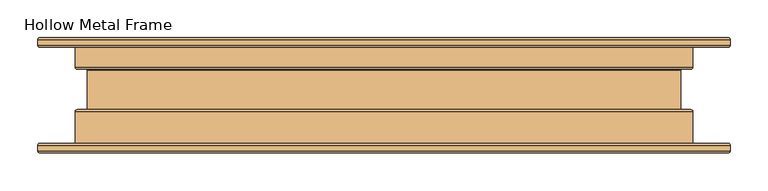
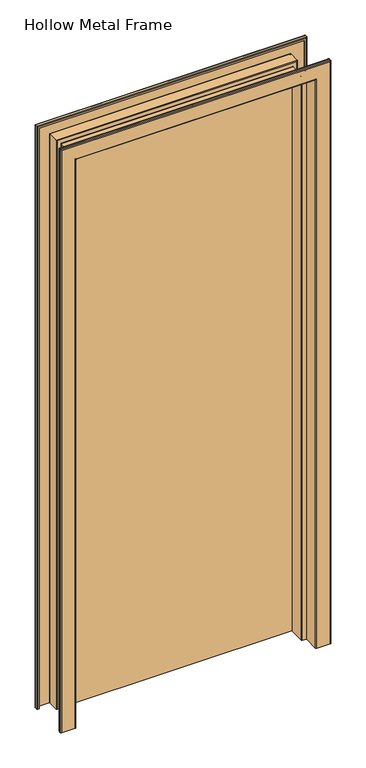
"""IFC4 building model written with IfcOpenShell, lengths in millimetres: door geometry, Hollow Metal Frame."""

from ifc_helpers import new_model, si_unit, frame, origin, origin_with_axes, place, context, project, spatial, polyline, circle_curve, ellipse_curve, outline, extrude, source, transform, mapped, element, save
from ifc_brep_helpers import plane_surface, cylinder_surface, revolved_surface, advanced_brep


def hollow_metal_frame_df2d566d(model_context):
    return source(origin(), model_context, "Body", "SolidModel", [
        advanced_brep(
        [(-454.62825, -63.5635, 0.0), (-449.2625, -63.5635, 0.0), (-449.2625, -65.11925, 0.0), (-454.62825, -65.11925, 0.0), (-455.64425, -66.13525, 0.0), (-455.64425, -73.66, 0.0), (-454.62825, -74.676, 0.0), (-408.97175, -74.676, 0.0), (-407.95575, -73.66, 0.0), (-407.95575, -21.68525, 0.0), (-405.384, -19.1135, 0.0), (-393.09675, -19.1135, 0.0), (-392.08075, -18.0975, 0.0), (-392.08075, 33.6931, 0.0), (-393.09675, 34.7091, 0.0), (-405.384, 34.7091, 0.0), (-407.95575, 37.28085, 0.0), (-407.95575, 73.5965, 0.0), (-408.97175, 74.6125, 0.0), (-454.62825, 74.6125, 0.0), (-455.64425, 73.5965, 0.0), (-455.64425, 66.07175, 0.0), (-454.62825, 65.05575, 0.0), (-449.2625, 65.05575, 0.0), (-449.2625, 63.5, 0.0), (-454.62825, 63.5, 0.0), (-457.2, 66.07175, 0.0), (-457.2, 73.5965, 0.0), (-454.62825, 76.16825, 0.0), (-408.97175, 76.16825, 0.0), (-406.4, 73.5965, 0.0), (-406.4, 37.28085, 0.0), (-405.384, 36.26485, 0.0), (-393.09675, 36.26485, 0.0), (-390.525, 33.6931, 0.0), (-390.525, -18.0975, 0.0), (-393.09675, -20.66925, 0.0), (-405.384, -20.66925, 0.0), (-406.4, -21.68525, 0.0), (-406.4, -73.66, 0.0), (-408.97175, -76.23175, 0.0), (-454.62825, -76.23175, 0.0), (-457.2, -73.66, 0.0), (-457.2, -66.13525, 0.0), (-457.2, -66.13525, 2082.8000001), (-454.62825, -63.5635, 2080.2282501), (-457.2, -73.66, 2082.8000001), (-454.62825, -76.23175, 2080.2282501), (-408.97175, -76.23175, 2034.5717501), (408.97175, -76.23175, 2034.5717501), (408.97175, -76.23175, 0.0), (454.62825, -76.23175, 0.0), (454.62825, -76.23175, 2080.2282501), (-406.4, -73.66, 2032.0000001), (-406.4, -21.68525, 2032.0000001), (-405.384, -20.66925, 2030.9840001), (-393.09675, -20.66925, 2018.6967501), (393.09675, -20.66925, 2018.6967501), (393.09675, -20.66925, 0.0), (405.384, -20.66925, 0.0), (405.384, -20.66925, 2030.9840001), (-390.525, -18.0975, 2016.1250001), (-390.525, 33.6931, 2016.1250001), (-393.09675, 36.26485, 2018.6967501), (-405.384, 36.26485, 2030.9840001), (405.384, 36.26485, 2030.9840001), (405.384, 36.26485, 0.0), (393.09675, 36.26485, 0.0), (393.09675, 36.26485, 2018.6967501), (-406.4, 37.28085, 2032.0000001), (-406.4, 73.5965, 2032.0000001), (-408.97175, 76.16825, 2034.5717501), (-454.62825, 76.16825, 2080.2282501), (454.62825, 76.16825, 2080.2282501), (454.62825, 76.16825, 0.0), (408.97175, 76.16825, 0.0), (408.97175, 76.16825, 2034.5717501), (-457.2, 73.5965, 2082.8000001), (-457.2, 66.07175, 2082.8000001), (-454.62825, 63.5, 2080.2282501), (-449.2625, 63.5, 2074.8625001), (449.2625, 63.5, 2074.8625001), (449.2625, 63.5, 0.0), (454.62825, 63.5, 0.0), (454.62825, 63.5, 2080.2282501), (-449.2625, 65.05575, 2074.8625001), (-454.62825, 65.05575, 2080.2282501), (454.62825, 65.05575, 2080.2282501), (454.62825, 65.05575, 0.0), (449.2625, 65.05575, 0.0), (449.2625, 65.05575, 2074.8625001), (-455.64425, 66.07175, 2081.2442501), (-455.64425, 73.5965, 2081.2442501), (-454.62825, 74.6125, 2080.2282501), (-408.97175, 74.6125, 2034.5717501), (408.97175, 74.6125, 2034.5717501), (408.97175, 74.6125, 0.0), (454.62825, 74.6125, 0.0), (454.62825, 74.6125, 2080.2282501), (-407.95575, 73.5965, 2033.5557501), (-407.95575, 37.28085, 2033.5557501), (-405.384, 34.7091, 2030.9840001), (-393.09675, 34.7091, 2018.6967501), (393.09675, 34.7091, 2018.6967501), (393.09675, 34.7091, 0.0), (405.384, 34.7091, 0.0), (405.384, 34.7091, 2030.9840001), (-392.08075, 33.6931, 2017.6807501), (-392.08075, -18.0975, 2017.6807501), (-393.09675, -19.1135, 2018.6967501), (-405.384, -19.1135, 2030.9840001), (405.384, -19.1135, 2030.9840001), (405.384, -19.1135, 0.0), (393.09675, -19.1135, 0.0), (393.09675, -19.1135, 2018.6967501), (-407.95575, -21.68525, 2033.5557501), (-407.95575, -73.66, 2033.5557501), (-408.97175, -74.676, 2034.5717501), (-454.62825, -74.676, 2080.2282501), (454.62825, -74.676, 2080.2282501), (454.62825, -74.676, 0.0), (408.97175, -74.676, 0.0), (408.97175, -74.676, 2034.5717501), (-455.64425, -73.66, 2081.2442501), (-455.64425, -66.13525, 2081.2442501), (-454.62825, -65.11925, 2080.2282501), (-449.2625, -65.11925, 2074.8625001), (449.2625, -65.11925, 2074.8625001), (449.2625, -65.11925, 0.0), (454.62825, -65.11925, 0.0), (454.62825, -65.11925, 2080.2282501), (-449.2625, -63.5635, 2074.8625001), (454.62825, -63.5635, 2080.2282501), (454.62825, -63.5635, 0.0), (449.2625, -63.5635, 0.0), (449.2625, -63.5635, 2074.8625001), (457.2, -66.13525, 2082.8000001), (457.2, -73.66, 2082.8000001), (406.4, -73.66, 2032.0000001), (406.4, -21.68525, 2032.0000001), (390.525, -18.0975, 2016.1250001), (390.525, 33.6931, 2016.1250001), (406.4, 37.28085, 2032.0000001), (406.4, 73.5965, 2032.0000001), (457.2, 73.5965, 2082.8000001), (457.2, 66.07175, 2082.8000001), (455.64425, 66.07175, 2081.2442501), (455.64425, 73.5965, 2081.2442501), (407.95575, 73.5965, 2033.5557501), (407.95575, 37.28085, 2033.5557501), (392.08075, 33.6931, 2017.6807501), (392.08075, -18.0975, 2017.6807501), (407.95575, -21.68525, 2033.5557501), (407.95575, -73.66, 2033.5557501), (455.64425, -73.66, 2081.2442501), (455.64425, -66.13525, 2081.2442501), (457.2, -66.13525, 0.0), (457.2, -73.66, 0.0), (406.4, -73.66, 0.0), (406.4, -21.68525, 0.0), (390.525, -18.0975, 0.0), (390.525, 33.6931, 0.0), (406.4, 37.28085, 0.0), (406.4, 73.5965, 0.0), (457.2, 73.5965, 0.0), (457.2, 66.07175, 0.0), (455.64425, 66.07175, 0.0), (455.64425, 73.5965, 0.0), (407.95575, 73.5965, 0.0), (407.95575, 37.28085, 0.0), (392.08075, 33.6931, 0.0), (392.08075, -18.0975, 0.0), (407.95575, -21.68525, 0.0), (407.95575, -73.66, 0.0), (455.64425, -73.66, 0.0), (455.64425, -66.13525, 0.0)],
        [
            (0, 1),
            (1, 2),
            (2, 3),
            (3, 4, circle_curve(frame((-454.62825, -66.13525, 0.0), z_axis=(0.0, 0.0, 1.0), x_axis=(0.0, 1.0, 0.0)), 1.016)),
            (4, 5),
            (5, 6, circle_curve(frame((-454.62825, -73.66, 0.0), z_axis=(0.0, 0.0, 1.0), x_axis=(0.0, 1.0, 0.0)), 1.016)),
            (6, 7),
            (7, 8, circle_curve(frame((-408.97175, -73.66, 0.0), z_axis=(0.0, 0.0, 1.0), x_axis=(0.0, 1.0, 0.0)), 1.016)),
            (8, 9),
            (9, 10, circle_curve(frame((-405.384, -21.68525, 0.0), z_axis=(0.0, 0.0, -1.0), x_axis=(0.0, 1.0, 0.0)), 2.57175)),
            (10, 11),
            (11, 12, circle_curve(frame((-393.09675, -18.0975, 0.0), z_axis=(0.0, 0.0, 1.0), x_axis=(0.0, 1.0, 0.0)), 1.016)),
            (12, 13),
            (13, 14, circle_curve(frame((-393.09675, 33.6931, 0.0), z_axis=(0.0, 0.0, 1.0), x_axis=(0.0, 1.0, 0.0)), 1.016)),
            (14, 15),
            (15, 16, circle_curve(frame((-405.384, 37.28085, 0.0), z_axis=(0.0, 0.0, -1.0), x_axis=(0.0, 1.0, 0.0)), 2.57175)),
            (16, 17),
            (17, 18, circle_curve(frame((-408.97175, 73.5965, 0.0), z_axis=(0.0, 0.0, 1.0), x_axis=(0.0, 1.0, 0.0)), 1.016)),
            (18, 19),
            (19, 20, circle_curve(frame((-454.62825, 73.5965, 0.0), z_axis=(0.0, 0.0, 1.0), x_axis=(0.0, 1.0, 0.0)), 1.016)),
            (20, 21),
            (21, 22, circle_curve(frame((-454.62825, 66.07175, 0.0), z_axis=(0.0, 0.0, 1.0), x_axis=(0.0, 1.0, 0.0)), 1.016)),
            (22, 23),
            (23, 24),
            (24, 25),
            (25, 26, circle_curve(frame((-454.62825, 66.07175, 0.0), z_axis=(0.0, 0.0, -1.0), x_axis=(0.0, 1.0, 0.0)), 2.57175)),
            (26, 27),
            (27, 28, circle_curve(frame((-454.62825, 73.5965, 0.0), z_axis=(0.0, 0.0, -1.0), x_axis=(0.0, 1.0, 0.0)), 2.57175)),
            (28, 29),
            (29, 30, circle_curve(frame((-408.97175, 73.5965, 0.0), z_axis=(0.0, 0.0, -1.0), x_axis=(0.0, 1.0, 0.0)), 2.57175)),
            (30, 31),
            (31, 32, circle_curve(frame((-405.384, 37.28085, 0.0), z_axis=(0.0, 0.0, 1.0), x_axis=(0.0, 1.0, 0.0)), 1.016)),
            (32, 33),
            (33, 34, circle_curve(frame((-393.09675, 33.6931, 0.0), z_axis=(0.0, 0.0, -1.0), x_axis=(0.0, 1.0, 0.0)), 2.57175)),
            (34, 35),
            (35, 36, circle_curve(frame((-393.09675, -18.0975, 0.0), z_axis=(0.0, 0.0, -1.0), x_axis=(0.0, 1.0, 0.0)), 2.57175)),
            (36, 37),
            (37, 38, circle_curve(frame((-405.384, -21.68525, 0.0), z_axis=(0.0, 0.0, 1.0), x_axis=(0.0, 1.0, 0.0)), 1.016)),
            (38, 39),
            (39, 40, circle_curve(frame((-408.97175, -73.66, 0.0), z_axis=(0.0, 0.0, -1.0), x_axis=(0.0, 1.0, 0.0)), 2.57175)),
            (40, 41),
            (41, 42, circle_curve(frame((-454.62825, -73.66, 0.0), z_axis=(0.0, 0.0, -1.0), x_axis=(0.0, 1.0, 0.0)), 2.57175)),
            (42, 43),
            (43, 0, circle_curve(frame((-454.62825, -66.13525, 0.0), z_axis=(0.0, 0.0, -1.0), x_axis=(0.0, 1.0, 0.0)), 2.57175)),
            (43, 44),
            (44, 45, ellipse_curve(frame((-454.62825, -66.13525, 2080.2282501), z_axis=(-0.7071067811865475, 0.0, -0.7071067811865475), x_axis=(0.7071067811865474, 0.0, -0.7071067811865476)), 3.6370037, 2.57175)),
            (45, 0),
            (42, 46),
            (46, 44),
            (41, 47),
            (47, 46, ellipse_curve(frame((-454.62825, -73.66, 2080.2282501), z_axis=(-0.7071067811865475, 0.0, -0.7071067811865475), x_axis=(0.7071067811865474, 0.0, -0.7071067811865476)), 3.6370037, 2.57175)),
            (40, 48),
            (48, 49),
            (49, 50),
            (50, 51),
            (51, 52),
            (52, 47),
            (39, 53),
            (53, 48, ellipse_curve(frame((-408.97175, -73.66, 2034.5717501), z_axis=(-0.7071067811865475, 0.0, -0.7071067811865475), x_axis=(0.7071067811865474, 0.0, -0.7071067811865476)), 3.6370037, 2.57175)),
            (38, 54),
            (54, 53),
            (37, 55),
            (55, 54, ellipse_curve(frame((-405.384, -21.68525, 2030.9840001), z_axis=(0.7071067811865475, 0.0, 0.7071067811865475), x_axis=(-0.7071067811865474, 0.0, 0.7071067811865476)), 1.436841, 1.016)),
            (36, 56),
            (56, 57),
            (57, 58),
            (58, 59),
            (59, 60),
            (60, 55),
            (35, 61),
            (61, 56, ellipse_curve(frame((-393.09675, -18.0975, 2018.6967501), z_axis=(-0.7071067811865475, 0.0, -0.7071067811865475), x_axis=(0.7071067811865474, 0.0, -0.7071067811865476)), 3.6370037, 2.57175)),
            (34, 62),
            (62, 61),
            (33, 63),
            (63, 62, ellipse_curve(frame((-393.09675, 33.6931, 2018.6967501), z_axis=(-0.7071067811865475, 0.0, -0.7071067811865475), x_axis=(0.7071067811865474, 0.0, -0.7071067811865476)), 3.6370037, 2.57175)),
            (32, 64),
            (64, 65),
            (65, 66),
            (66, 67),
            (67, 68),
            (68, 63),
            (31, 69),
            (69, 64, ellipse_curve(frame((-405.384, 37.28085, 2030.9840001), z_axis=(0.7071067811865475, 0.0, 0.7071067811865475), x_axis=(-0.7071067811865474, 0.0, 0.7071067811865476)), 1.436841, 1.016)),
            (30, 70),
            (70, 69),
            (29, 71),
            (71, 70, ellipse_curve(frame((-408.97175, 73.5965, 2034.5717501), z_axis=(-0.7071067811865475, 0.0, -0.7071067811865475), x_axis=(0.7071067811865474, 0.0, -0.7071067811865476)), 3.6370037, 2.57175)),
            (28, 72),
            (72, 73),
            (73, 74),
            (74, 75),
            (75, 76),
            (76, 71),
            (27, 77),
            (77, 72, ellipse_curve(frame((-454.62825, 73.5965, 2080.2282501), z_axis=(-0.7071067811865475, 0.0, -0.7071067811865475), x_axis=(0.7071067811865474, 0.0, -0.7071067811865476)), 3.6370037, 2.57175)),
            (26, 78),
            (78, 77),
            (25, 79),
            (79, 78, ellipse_curve(frame((-454.62825, 66.07175, 2080.2282501), z_axis=(-0.7071067811865475, 0.0, -0.7071067811865475), x_axis=(0.7071067811865474, 0.0, -0.7071067811865476)), 3.6370037, 2.57175)),
            (24, 80),
            (80, 81),
            (81, 82),
            (82, 83),
            (83, 84),
            (84, 79),
            (23, 85),
            (85, 80),
            (22, 86),
            (86, 87),
            (87, 88),
            (88, 89),
            (89, 90),
            (90, 85),
            (21, 91),
            (91, 86, ellipse_curve(frame((-454.62825, 66.07175, 2080.2282501), z_axis=(0.7071067811865475, 0.0, 0.7071067811865475), x_axis=(-0.7071067811865474, 0.0, 0.7071067811865476)), 1.436841, 1.016)),
            (20, 92),
            (92, 91),
            (19, 93),
            (93, 92, ellipse_curve(frame((-454.62825, 73.5965, 2080.2282501), z_axis=(0.7071067811865475, 0.0, 0.7071067811865475), x_axis=(-0.7071067811865474, 0.0, 0.7071067811865476)), 1.436841, 1.016)),
            (18, 94),
            (94, 95),
            (95, 96),
            (96, 97),
            (97, 98),
            (98, 93),
            (17, 99),
            (99, 94, ellipse_curve(frame((-408.97175, 73.5965, 2034.5717501), z_axis=(0.7071067811865475, 0.0, 0.7071067811865475), x_axis=(-0.7071067811865474, 0.0, 0.7071067811865476)), 1.436841, 1.016)),
            (16, 100),
            (100, 99),
            (15, 101),
            (101, 100, ellipse_curve(frame((-405.384, 37.28085, 2030.9840001), z_axis=(-0.7071067811865475, 0.0, -0.7071067811865475), x_axis=(0.7071067811865474, 0.0, -0.7071067811865476)), 3.6370037, 2.57175)),
            (14, 102),
            (102, 103),
            (103, 104),
            (104, 105),
            (105, 106),
            (106, 101),
            (13, 107),
            (107, 102, ellipse_curve(frame((-393.09675, 33.6931, 2018.6967501), z_axis=(0.7071067811865475, 0.0, 0.7071067811865475), x_axis=(-0.7071067811865474, 0.0, 0.7071067811865476)), 1.436841, 1.016)),
            (12, 108),
            (108, 107),
            (11, 109),
            (109, 108, ellipse_curve(frame((-393.09675, -18.0975, 2018.6967501), z_axis=(0.7071067811865475, 0.0, 0.7071067811865475), x_axis=(-0.7071067811865474, 0.0, 0.7071067811865476)), 1.436841, 1.016)),
            (10, 110),
            (110, 111),
            (111, 112),
            (112, 113),
            (113, 114),
            (114, 109),
            (9, 115),
            (115, 110, ellipse_curve(frame((-405.384, -21.68525, 2030.9840001), z_axis=(-0.7071067811865475, 0.0, -0.7071067811865475), x_axis=(0.7071067811865474, 0.0, -0.7071067811865476)), 3.6370037, 2.57175)),
            (8, 116),
            (116, 115),
            (7, 117),
            (117, 116, ellipse_curve(frame((-408.97175, -73.66, 2034.5717501), z_axis=(0.7071067811865475, 0.0, 0.7071067811865475), x_axis=(-0.7071067811865474, 0.0, 0.7071067811865476)), 1.436841, 1.016)),
            (6, 118),
            (118, 119),
            (119, 120),
            (120, 121),
            (121, 122),
            (122, 117),
            (5, 123),
            (123, 118, ellipse_curve(frame((-454.62825, -73.66, 2080.2282501), z_axis=(0.7071067811865475, 0.0, 0.7071067811865475), x_axis=(-0.7071067811865474, 0.0, 0.7071067811865476)), 1.436841, 1.016)),
            (4, 124),
            (124, 123),
            (3, 125),
            (125, 124, ellipse_curve(frame((-454.62825, -66.13525, 2080.2282501), z_axis=(0.7071067811865475, 0.0, 0.7071067811865475), x_axis=(-0.7071067811865474, 0.0, 0.7071067811865476)), 1.436841, 1.016)),
            (2, 126),
            (126, 127),
            (127, 128),
            (128, 129),
            (129, 130),
            (130, 125),
            (1, 131),
            (131, 126),
            (45, 132),
            (132, 133),
            (133, 134),
            (134, 135),
            (135, 131),
            (44, 136),
            (136, 132, ellipse_curve(frame((454.62825, -66.13525, 2080.2282501), z_axis=(-0.7071067811865475, 0.0, 0.7071067811865475), x_axis=(-0.7071067811865476, 0.0, -0.7071067811865474)), 3.6370037, 2.57175)),
            (46, 137),
            (137, 136),
            (52, 137, ellipse_curve(frame((454.62825, -73.66, 2080.2282501), z_axis=(-0.7071067811865475, 0.0, 0.7071067811865475), x_axis=(-0.7071067811865476, 0.0, -0.7071067811865474)), 3.6370037, 2.57175)),
            (53, 138),
            (138, 49, ellipse_curve(frame((408.97175, -73.66, 2034.5717501), z_axis=(-0.7071067811865475, 0.0, 0.7071067811865475), x_axis=(-0.7071067811865476, 0.0, -0.7071067811865474)), 3.6370037, 2.57175)),
            (54, 139),
            (139, 138),
            (60, 139, ellipse_curve(frame((405.384, -21.68525, 2030.9840001), z_axis=(0.7071067811865475, 0.0, -0.7071067811865475), x_axis=(0.7071067811865476, 0.0, 0.7071067811865474)), 1.436841, 1.016)),
            (61, 140),
            (140, 57, ellipse_curve(frame((393.09675, -18.0975, 2018.6967501), z_axis=(-0.7071067811865475, 0.0, 0.7071067811865475), x_axis=(-0.7071067811865476, 0.0, -0.7071067811865474)), 3.6370037, 2.57175)),
            (62, 141),
            (141, 140),
            (68, 141, ellipse_curve(frame((393.09675, 33.6931, 2018.6967501), z_axis=(-0.7071067811865475, 0.0, 0.7071067811865475), x_axis=(-0.7071067811865476, 0.0, -0.7071067811865474)), 3.6370037, 2.57175)),
            (69, 142),
            (142, 65, ellipse_curve(frame((405.384, 37.28085, 2030.9840001), z_axis=(0.7071067811865475, 0.0, -0.7071067811865475), x_axis=(0.7071067811865476, 0.0, 0.7071067811865474)), 1.436841, 1.016)),
            (70, 143),
            (143, 142),
            (76, 143, ellipse_curve(frame((408.97175, 73.5965, 2034.5717501), z_axis=(-0.7071067811865475, 0.0, 0.7071067811865475), x_axis=(-0.7071067811865476, 0.0, -0.7071067811865474)), 3.6370037, 2.57175)),
            (77, 144),
            (144, 73, ellipse_curve(frame((454.62825, 73.5965, 2080.2282501), z_axis=(-0.7071067811865475, 0.0, 0.7071067811865475), x_axis=(-0.7071067811865476, 0.0, -0.7071067811865474)), 3.6370037, 2.57175)),
            (78, 145),
            (145, 144),
            (84, 145, ellipse_curve(frame((454.62825, 66.07175, 2080.2282501), z_axis=(-0.7071067811865475, 0.0, 0.7071067811865475), x_axis=(-0.7071067811865476, 0.0, -0.7071067811865474)), 3.6370037, 2.57175)),
            (90, 81),
            (91, 146),
            (146, 87, ellipse_curve(frame((454.62825, 66.07175, 2080.2282501), z_axis=(0.7071067811865475, 0.0, -0.7071067811865475), x_axis=(0.7071067811865476, 0.0, 0.7071067811865474)), 1.436841, 1.016)),
            (92, 147),
            (147, 146),
            (98, 147, ellipse_curve(frame((454.62825, 73.5965, 2080.2282501), z_axis=(0.7071067811865475, 0.0, -0.7071067811865475), x_axis=(0.7071067811865476, 0.0, 0.7071067811865474)), 1.436841, 1.016)),
            (99, 148),
            (148, 95, ellipse_curve(frame((408.97175, 73.5965, 2034.5717501), z_axis=(0.7071067811865475, 0.0, -0.7071067811865475), x_axis=(0.7071067811865476, 0.0, 0.7071067811865474)), 1.436841, 1.016)),
            (100, 149),
            (149, 148),
            (106, 149, ellipse_curve(frame((405.384, 37.28085, 2030.9840001), z_axis=(-0.7071067811865475, 0.0, 0.7071067811865475), x_axis=(-0.7071067811865476, 0.0, -0.7071067811865474)), 3.6370037, 2.57175)),
            (107, 150),
            (150, 103, ellipse_curve(frame((393.09675, 33.6931, 2018.6967501), z_axis=(0.7071067811865475, 0.0, -0.7071067811865475), x_axis=(0.7071067811865476, 0.0, 0.7071067811865474)), 1.436841, 1.016)),
            (108, 151),
            (151, 150),
            (114, 151, ellipse_curve(frame((393.09675, -18.0975, 2018.6967501), z_axis=(0.7071067811865475, 0.0, -0.7071067811865475), x_axis=(0.7071067811865476, 0.0, 0.7071067811865474)), 1.436841, 1.016)),
            (115, 152),
            (152, 111, ellipse_curve(frame((405.384, -21.68525, 2030.9840001), z_axis=(-0.7071067811865475, 0.0, 0.7071067811865475), x_axis=(-0.7071067811865476, 0.0, -0.7071067811865474)), 3.6370037, 2.57175)),
            (116, 153),
            (153, 152),
            (122, 153, ellipse_curve(frame((408.97175, -73.66, 2034.5717501), z_axis=(0.7071067811865475, 0.0, -0.7071067811865475), x_axis=(0.7071067811865476, 0.0, 0.7071067811865474)), 1.436841, 1.016)),
            (123, 154),
            (154, 119, ellipse_curve(frame((454.62825, -73.66, 2080.2282501), z_axis=(0.7071067811865475, 0.0, -0.7071067811865475), x_axis=(0.7071067811865476, 0.0, 0.7071067811865474)), 1.436841, 1.016)),
            (124, 155),
            (155, 154),
            (130, 155, ellipse_curve(frame((454.62825, -66.13525, 2080.2282501), z_axis=(0.7071067811865475, 0.0, -0.7071067811865475), x_axis=(0.7071067811865476, 0.0, 0.7071067811865474)), 1.436841, 1.016)),
            (135, 127),
            (133, 156, circle_curve(frame((454.62825, -66.13525, 0.0), z_axis=(0.0, 0.0, -1.0), x_axis=(0.0, 1.0, 0.0)), 2.57175)),
            (156, 157),
            (157, 51, circle_curve(frame((454.62825, -73.66, 0.0), z_axis=(0.0, 0.0, -1.0), x_axis=(0.0, 1.0, 0.0)), 2.57175)),
            (50, 158, circle_curve(frame((408.97175, -73.66, 0.0), z_axis=(0.0, 0.0, -1.0), x_axis=(0.0, 1.0, 0.0)), 2.57175)),
            (158, 159),
            (159, 59, circle_curve(frame((405.384, -21.68525, 0.0), z_axis=(0.0, 0.0, 1.0), x_axis=(0.0, 1.0, 0.0)), 1.016)),
            (58, 160, circle_curve(frame((393.09675, -18.0975, 0.0), z_axis=(0.0, 0.0, -1.0), x_axis=(0.0, 1.0, 0.0)), 2.57175)),
            (160, 161),
            (161, 67, circle_curve(frame((393.09675, 33.6931, 0.0), z_axis=(0.0, 0.0, -1.0), x_axis=(0.0, 1.0, 0.0)), 2.57175)),
            (66, 162, circle_curve(frame((405.384, 37.28085, 0.0), z_axis=(0.0, 0.0, 1.0), x_axis=(0.0, 1.0, 0.0)), 1.016)),
            (162, 163),
            (163, 75, circle_curve(frame((408.97175, 73.5965, 0.0), z_axis=(0.0, 0.0, -1.0), x_axis=(0.0, 1.0, 0.0)), 2.57175)),
            (74, 164, circle_curve(frame((454.62825, 73.5965, 0.0), z_axis=(0.0, 0.0, -1.0), x_axis=(0.0, 1.0, 0.0)), 2.57175)),
            (164, 165),
            (165, 83, circle_curve(frame((454.62825, 66.07175, 0.0), z_axis=(0.0, 0.0, -1.0), x_axis=(0.0, 1.0, 0.0)), 2.57175)),
            (82, 89),
            (88, 166, circle_curve(frame((454.62825, 66.07175, 0.0), z_axis=(0.0, 0.0, 1.0), x_axis=(0.0, 1.0, 0.0)), 1.016)),
            (166, 167),
            (167, 97, circle_curve(frame((454.62825, 73.5965, 0.0), z_axis=(0.0, 0.0, 1.0), x_axis=(0.0, 1.0, 0.0)), 1.016)),
            (96, 168, circle_curve(frame((408.97175, 73.5965, 0.0), z_axis=(0.0, 0.0, 1.0), x_axis=(0.0, 1.0, 0.0)), 1.016)),
            (168, 169),
            (169, 105, circle_curve(frame((405.384, 37.28085, 0.0), z_axis=(0.0, 0.0, -1.0), x_axis=(0.0, 1.0, 0.0)), 2.57175)),
            (104, 170, circle_curve(frame((393.09675, 33.6931, 0.0), z_axis=(0.0, 0.0, 1.0), x_axis=(0.0, 1.0, 0.0)), 1.016)),
            (170, 171),
            (171, 113, circle_curve(frame((393.09675, -18.0975, 0.0), z_axis=(0.0, 0.0, 1.0), x_axis=(0.0, 1.0, 0.0)), 1.016)),
            (112, 172, circle_curve(frame((405.384, -21.68525, 0.0), z_axis=(0.0, 0.0, -1.0), x_axis=(0.0, 1.0, 0.0)), 2.57175)),
            (172, 173),
            (173, 121, circle_curve(frame((408.97175, -73.66, 0.0), z_axis=(0.0, 0.0, 1.0), x_axis=(0.0, 1.0, 0.0)), 1.016)),
            (120, 174, circle_curve(frame((454.62825, -73.66, 0.0), z_axis=(0.0, 0.0, 1.0), x_axis=(0.0, 1.0, 0.0)), 1.016)),
            (174, 175),
            (175, 129, circle_curve(frame((454.62825, -66.13525, 0.0), z_axis=(0.0, 0.0, 1.0), x_axis=(0.0, 1.0, 0.0)), 1.016)),
            (128, 134),
            (136, 156),
            (137, 157),
            (138, 158),
            (139, 159),
            (140, 160),
            (141, 161),
            (142, 162),
            (143, 163),
            (144, 164),
            (145, 165),
            (146, 166),
            (147, 167),
            (148, 168),
            (149, 169),
            (150, 170),
            (151, 171),
            (152, 172),
            (153, 173),
            (154, 174),
            (155, 175),
        ],
        [
            plane_surface(frame((-417.5125, 63.5, 0.0), z_axis=(0.0, 0.0, -1.0), x_axis=(1.0, 0.0, 0.0))),
            cylinder_surface(frame((-454.62825, -66.13525, 0.0), z_axis=(0.0, 0.0, -1.0), x_axis=(0.0, 1.0, 0.0)), 2.57175),
            plane_surface(frame((-457.2, -66.13525, 0.0), z_axis=(-1.0, 0.0, 0.0), x_axis=(0.0, 0.0, 1.0))),
            cylinder_surface(frame((-454.62825, -73.66, 0.0), z_axis=(0.0, 0.0, -1.0), x_axis=(0.0, 1.0, 0.0)), 2.57175),
            plane_surface(frame((-454.62825, -76.23175, 0.0), z_axis=(0.0, -1.0, 0.0), x_axis=(0.0, 0.0, 1.0))),
            cylinder_surface(frame((-408.97175, -73.66, 0.0), z_axis=(0.0, 0.0, -1.0), x_axis=(0.0, 1.0, 0.0)), 2.57175),
            plane_surface(frame((-406.4, -73.66, 0.0), z_axis=(1.0, 0.0, 0.0), x_axis=(0.0, 0.0, 1.0))),
            revolved_surface(polyline([(-405.384, -20.669249999999998, 2032.0000001145868), (-405.384, -20.669249999999998, 0.0)]), (-405.384, -21.68525, 0.0), (0.0, 0.0, 1.0)),
            plane_surface(frame((-405.384, -20.66925, 0.0), z_axis=(0.0, -1.0, 0.0), x_axis=(0.0, 0.0, 1.0))),
            cylinder_surface(frame((-393.09675, -18.0975, 0.0), z_axis=(0.0, 0.0, -1.0), x_axis=(0.0, 1.0, 0.0)), 2.57175),
            plane_surface(frame((-390.525, -18.0975, 0.0), z_axis=(1.0, 0.0, 0.0), x_axis=(0.0, 0.0, 1.0))),
            cylinder_surface(frame((-393.09675, 33.6931, 0.0), z_axis=(0.0, 0.0, -1.0), x_axis=(0.0, 1.0, 0.0)), 2.57175),
            plane_surface(frame((-393.09675, 36.26485, 0.0), z_axis=(0.0, 1.0, 0.0), x_axis=(0.0, 0.0, 1.0))),
            revolved_surface(polyline([(-405.384, 38.29685, 2032.0000001145868), (-405.384, 38.29685, 0.0)]), (-405.384, 37.28085, 0.0), (0.0, 0.0, 1.0)),
            plane_surface(frame((-406.4, 37.28085, 0.0), z_axis=(1.0, 0.0, 0.0), x_axis=(0.0, 0.0, 1.0))),
            cylinder_surface(frame((-408.97175, 73.5965, 0.0), z_axis=(0.0, 0.0, -1.0), x_axis=(0.0, 1.0, 0.0)), 2.57175),
            plane_surface(frame((-408.97175, 76.16825, 0.0), z_axis=(0.0, 1.0, 0.0), x_axis=(0.0, 0.0, 1.0))),
            cylinder_surface(frame((-454.62825, 73.5965, 0.0), z_axis=(0.0, 0.0, -1.0), x_axis=(0.0, 1.0, 0.0)), 2.57175),
            plane_surface(frame((-457.2, 73.5965, 0.0), z_axis=(-1.0, 0.0, 0.0), x_axis=(0.0, 0.0, 1.0))),
            cylinder_surface(frame((-454.62825, 66.07175, 0.0), z_axis=(0.0, 0.0, -1.0), x_axis=(0.0, 1.0, 0.0)), 2.57175),
            plane_surface(frame((-454.62825, 63.5, 0.0), z_axis=(0.0, -1.0, 0.0), x_axis=(0.0, 0.0, 1.0))),
            plane_surface(frame((-449.2625, 63.5, 0.0), z_axis=(1.0, 0.0, 0.0), x_axis=(0.0, 0.0, 1.0))),
            plane_surface(frame((-449.2625, 65.05575, 0.0), z_axis=(0.0, 1.0, 0.0), x_axis=(0.0, 0.0, 1.0))),
            revolved_surface(polyline([(-454.62825, 67.08775, 2081.244250114587), (-454.62825, 67.08775, 0.0)]), (-454.62825, 66.07175, 0.0), (0.0, 0.0, 1.0)),
            plane_surface(frame((-455.64425, 66.07175, 0.0), z_axis=(1.0, 0.0, 0.0), x_axis=(0.0, 0.0, 1.0))),
            revolved_surface(polyline([(-454.62825, 74.61250000000001, 2081.244250114587), (-454.62825, 74.61250000000001, 0.0)]), (-454.62825, 73.5965, 0.0), (0.0, 0.0, 1.0)),
            plane_surface(frame((-454.62825, 74.6125, 0.0), z_axis=(0.0, -1.0, 0.0), x_axis=(0.0, 0.0, 1.0))),
            revolved_surface(polyline([(-408.97175, 74.61250000000001, 2035.5877501145867), (-408.97175, 74.61250000000001, 0.0)]), (-408.97175, 73.5965, 0.0), (0.0, 0.0, 1.0)),
            plane_surface(frame((-407.95575, 73.5965, 0.0), z_axis=(-1.0, 0.0, 0.0), x_axis=(0.0, 0.0, 1.0))),
            cylinder_surface(frame((-405.384, 37.28085, 0.0), z_axis=(0.0, 0.0, -1.0), x_axis=(0.0, 1.0, 0.0)), 2.57175),
            plane_surface(frame((-405.384, 34.7091, 0.0), z_axis=(0.0, -1.0, 0.0), x_axis=(0.0, 0.0, 1.0))),
            revolved_surface(polyline([(-393.09675, 34.7091, 2019.7127501145867), (-393.09675, 34.7091, 0.0)]), (-393.09675, 33.6931, 0.0), (0.0, 0.0, 1.0)),
            plane_surface(frame((-392.08075, 33.6931, 0.0), z_axis=(-1.0, 0.0, 0.0), x_axis=(0.0, 0.0, 1.0))),
            revolved_surface(polyline([(-393.09675, -17.0815, 2019.7127501145867), (-393.09675, -17.0815, 0.0)]), (-393.09675, -18.0975, 0.0), (0.0, 0.0, 1.0)),
            plane_surface(frame((-393.09675, -19.1135, 0.0), z_axis=(0.0, 1.0, 0.0), x_axis=(0.0, 0.0, 1.0))),
            cylinder_surface(frame((-405.384, -21.68525, 0.0), z_axis=(0.0, 0.0, -1.0), x_axis=(0.0, 1.0, 0.0)), 2.57175),
            plane_surface(frame((-407.95575, -21.68525, 0.0), z_axis=(-1.0, 0.0, 0.0), x_axis=(0.0, 0.0, 1.0))),
            revolved_surface(polyline([(-408.97175, -72.64399999999999, 2035.5877501145867), (-408.97175, -72.64399999999999, 0.0)]), (-408.97175, -73.66, 0.0), (0.0, 0.0, 1.0)),
            plane_surface(frame((-408.97175, -74.676, 0.0), z_axis=(0.0, 1.0, 0.0), x_axis=(0.0, 0.0, 1.0))),
            revolved_surface(polyline([(-454.62825, -72.64399999999999, 2081.244250114587), (-454.62825, -72.64399999999999, 0.0)]), (-454.62825, -73.66, 0.0), (0.0, 0.0, 1.0)),
            plane_surface(frame((-455.64425, -73.66, 0.0), z_axis=(1.0, 0.0, 0.0), x_axis=(0.0, 0.0, 1.0))),
            revolved_surface(polyline([(-454.62825, -65.11925, 2081.244250114587), (-454.62825, -65.11925, 0.0)]), (-454.62825, -66.13525, 0.0), (0.0, 0.0, 1.0)),
            plane_surface(frame((-454.62825, -65.11925, 0.0), z_axis=(0.0, -1.0, 0.0), x_axis=(0.0, 0.0, 1.0))),
            plane_surface(frame((-449.2625, -65.11925, 0.0), z_axis=(1.0, 0.0, 0.0), x_axis=(0.0, 0.0, 1.0))),
            plane_surface(frame((-449.2625, -63.5635, 0.0), z_axis=(0.0, 1.0, 0.0), x_axis=(0.0, 0.0, 1.0))),
            cylinder_surface(frame((-417.5125, -66.13525, 2080.2282501), z_axis=(-1.0, 0.0, 0.0), x_axis=(0.0, 1.0, 0.0)), 2.57175),
            plane_surface(frame((-457.2, -66.13525, 2082.8000001), z_axis=(0.0, 0.0, 1.0), x_axis=(1.0, 0.0, 0.0))),
            cylinder_surface(frame((-417.5125, -73.66, 2080.2282501), z_axis=(-1.0, 0.0, 0.0), x_axis=(0.0, 1.0, 0.0)), 2.57175),
            cylinder_surface(frame((-417.5125, -73.66, 2034.5717501), z_axis=(-1.0, 0.0, 0.0), x_axis=(0.0, 1.0, 0.0)), 2.57175),
            plane_surface(frame((-406.4, -73.66, 2032.0000001), z_axis=(0.0, 0.0, -1.0), x_axis=(1.0, 0.0, 0.0))),
            revolved_surface(polyline([(406.40000001458696, -20.669249999999998, 2030.9840001), (-406.40000001458685, -20.669249999999998, 2030.9840001)]), (-417.5125, -21.68525, 2030.9840001), (1.0, 0.0, 0.0)),
            cylinder_surface(frame((-417.5125, -18.0975, 2018.6967501), z_axis=(-1.0, 0.0, 0.0), x_axis=(0.0, 1.0, 0.0)), 2.57175),
            plane_surface(frame((-390.525, -18.0975, 2016.1250001), z_axis=(0.0, 0.0, -1.0), x_axis=(1.0, 0.0, 0.0))),
            cylinder_surface(frame((-417.5125, 33.6931, 2018.6967501), z_axis=(-1.0, 0.0, 0.0), x_axis=(0.0, 1.0, 0.0)), 2.57175),
            revolved_surface(polyline([(406.40000001458696, 38.29685, 2030.9840001), (-406.40000001458685, 38.29685, 2030.9840001)]), (-417.5125, 37.28085, 2030.9840001), (1.0, 0.0, 0.0)),
            plane_surface(frame((-406.4, 37.28085, 2032.0000001), z_axis=(0.0, 0.0, -1.0), x_axis=(1.0, 0.0, 0.0))),
            cylinder_surface(frame((-417.5125, 73.5965, 2034.5717501), z_axis=(-1.0, 0.0, 0.0), x_axis=(0.0, 1.0, 0.0)), 2.57175),
            cylinder_surface(frame((-417.5125, 73.5965, 2080.2282501), z_axis=(-1.0, 0.0, 0.0), x_axis=(0.0, 1.0, 0.0)), 2.57175),
            plane_surface(frame((-457.2, 73.5965, 2082.8000001), z_axis=(0.0, 0.0, 1.0), x_axis=(1.0, 0.0, 0.0))),
            cylinder_surface(frame((-417.5125, 66.07175, 2080.2282501), z_axis=(-1.0, 0.0, 0.0), x_axis=(0.0, 1.0, 0.0)), 2.57175),
            plane_surface(frame((-449.2625, 63.5, 2074.8625001), z_axis=(0.0, 0.0, -1.0), x_axis=(1.0, 0.0, 0.0))),
            revolved_surface(polyline([(455.64425001458693, 67.08775, 2080.2282501), (-455.6442500145868, 67.08775, 2080.2282501)]), (-417.5125, 66.07175, 2080.2282501), (1.0, 0.0, 0.0)),
            plane_surface(frame((-455.64425, 66.07175, 2081.2442501), z_axis=(0.0, 0.0, -1.0), x_axis=(1.0, 0.0, 0.0))),
            revolved_surface(polyline([(455.64425001458693, 74.61250000000001, 2080.2282501), (-455.6442500145868, 74.61250000000001, 2080.2282501)]), (-417.5125, 73.5965, 2080.2282501), (1.0, 0.0, 0.0)),
            revolved_surface(polyline([(409.9877500145869, 74.61250000000001, 2034.5717501), (-409.9877500145868, 74.61250000000001, 2034.5717501)]), (-417.5125, 73.5965, 2034.5717501), (1.0, 0.0, 0.0)),
            plane_surface(frame((-407.95575, 73.5965, 2033.5557501), z_axis=(0.0, 0.0, 1.0), x_axis=(1.0, 0.0, 0.0))),
            cylinder_surface(frame((-417.5125, 37.28085, 2030.9840001), z_axis=(-1.0, 0.0, 0.0), x_axis=(0.0, 1.0, 0.0)), 2.57175),
            revolved_surface(polyline([(394.1127500145869, 34.7091, 2018.6967501), (-394.1127500145868, 34.7091, 2018.6967501)]), (-417.5125, 33.6931, 2018.6967501), (1.0, 0.0, 0.0)),
            plane_surface(frame((-392.08075, 33.6931, 2017.6807501), z_axis=(0.0, 0.0, 1.0), x_axis=(1.0, 0.0, 0.0))),
            revolved_surface(polyline([(394.1127500145869, -17.0815, 2018.6967501), (-394.1127500145868, -17.0815, 2018.6967501)]), (-417.5125, -18.0975, 2018.6967501), (1.0, 0.0, 0.0)),
            cylinder_surface(frame((-417.5125, -21.68525, 2030.9840001), z_axis=(-1.0, 0.0, 0.0), x_axis=(0.0, 1.0, 0.0)), 2.57175),
            plane_surface(frame((-407.95575, -21.68525, 2033.5557501), z_axis=(0.0, 0.0, 1.0), x_axis=(1.0, 0.0, 0.0))),
            revolved_surface(polyline([(409.9877500145869, -72.64399999999999, 2034.5717501), (-409.9877500145868, -72.64399999999999, 2034.5717501)]), (-417.5125, -73.66, 2034.5717501), (1.0, 0.0, 0.0)),
            revolved_surface(polyline([(455.64425001458693, -72.64399999999999, 2080.2282501), (-455.6442500145868, -72.64399999999999, 2080.2282501)]), (-417.5125, -73.66, 2080.2282501), (1.0, 0.0, 0.0)),
            plane_surface(frame((-455.64425, -73.66, 2081.2442501), z_axis=(0.0, 0.0, -1.0), x_axis=(1.0, 0.0, 0.0))),
            revolved_surface(polyline([(455.64425001458693, -65.11925, 2080.2282501), (-455.6442500145868, -65.11925, 2080.2282501)]), (-417.5125, -66.13525, 2080.2282501), (1.0, 0.0, 0.0)),
            plane_surface(frame((-449.2625, -65.11925, 2074.8625001), z_axis=(0.0, 0.0, -1.0), x_axis=(1.0, 0.0, 0.0))),
            plane_surface(frame((417.5125, 63.5, 0.0), z_axis=(0.0, 0.0, -1.0), x_axis=(-1.0, 0.0, 0.0))),
            cylinder_surface(frame((454.62825, -66.13525, 2043.1125001), z_axis=(0.0, 0.0, 1.0), x_axis=(0.0, 1.0, 0.0)), 2.57175),
            plane_surface(frame((457.2, -66.13525, 2082.8000001), z_axis=(1.0, 0.0, 0.0), x_axis=(0.0, 0.0, -1.0))),
            cylinder_surface(frame((454.62825, -73.66, 2043.1125001), z_axis=(0.0, 0.0, 1.0), x_axis=(0.0, 1.0, 0.0)), 2.57175),
            cylinder_surface(frame((408.97175, -73.66, 2043.1125001), z_axis=(0.0, 0.0, 1.0), x_axis=(0.0, 1.0, 0.0)), 2.57175),
            plane_surface(frame((406.4, -73.66, 2032.0000001), z_axis=(-1.0, 0.0, 0.0), x_axis=(0.0, 0.0, -1.0))),
            revolved_surface(polyline([(405.384, -20.669249999999998, 0.0), (405.384, -20.669249999999998, 2032.0000001145868)]), (405.384, -21.68525, 2043.1125001), (0.0, 0.0, -1.0)),
            cylinder_surface(frame((393.09675, -18.0975, 2043.1125001), z_axis=(0.0, 0.0, 1.0), x_axis=(0.0, 1.0, 0.0)), 2.57175),
            plane_surface(frame((390.525, -18.0975, 2016.1250001), z_axis=(-1.0, 0.0, 0.0), x_axis=(0.0, 0.0, -1.0))),
            cylinder_surface(frame((393.09675, 33.6931, 2043.1125001), z_axis=(0.0, 0.0, 1.0), x_axis=(0.0, 1.0, 0.0)), 2.57175),
            revolved_surface(polyline([(405.384, 38.29685, 0.0), (405.384, 38.29685, 2032.0000001145868)]), (405.384, 37.28085, 2043.1125001), (0.0, 0.0, -1.0)),
            plane_surface(frame((406.4, 37.28085, 2032.0000001), z_axis=(-1.0, 0.0, 0.0), x_axis=(0.0, 0.0, -1.0))),
            cylinder_surface(frame((408.97175, 73.5965, 2043.1125001), z_axis=(0.0, 0.0, 1.0), x_axis=(0.0, 1.0, 0.0)), 2.57175),
            cylinder_surface(frame((454.62825, 73.5965, 2043.1125001), z_axis=(0.0, 0.0, 1.0), x_axis=(0.0, 1.0, 0.0)), 2.57175),
            plane_surface(frame((457.2, 73.5965, 2082.8000001), z_axis=(1.0, 0.0, 0.0), x_axis=(0.0, 0.0, -1.0))),
            cylinder_surface(frame((454.62825, 66.07175, 2043.1125001), z_axis=(0.0, 0.0, 1.0), x_axis=(0.0, 1.0, 0.0)), 2.57175),
            plane_surface(frame((449.2625, 63.5, 2074.8625001), z_axis=(-1.0, 0.0, 0.0), x_axis=(0.0, 0.0, -1.0))),
            revolved_surface(polyline([(454.62825, 67.08775, 0.0), (454.62825, 67.08775, 2081.244250114587)]), (454.62825, 66.07175, 2043.1125001), (0.0, 0.0, -1.0)),
            plane_surface(frame((455.64425, 66.07175, 2081.2442501), z_axis=(-1.0, 0.0, 0.0), x_axis=(0.0, 0.0, -1.0))),
            revolved_surface(polyline([(454.62825, 74.61250000000001, 0.0), (454.62825, 74.61250000000001, 2081.244250114587)]), (454.62825, 73.5965, 2043.1125001), (0.0, 0.0, -1.0)),
            revolved_surface(polyline([(408.97175, 74.61250000000001, 0.0), (408.97175, 74.61250000000001, 2035.5877501145867)]), (408.97175, 73.5965, 2043.1125001), (0.0, 0.0, -1.0)),
            plane_surface(frame((407.95575, 73.5965, 2033.5557501), z_axis=(1.0, 0.0, 0.0), x_axis=(0.0, 0.0, -1.0))),
            cylinder_surface(frame((405.384, 37.28085, 2043.1125001), z_axis=(0.0, 0.0, 1.0), x_axis=(0.0, 1.0, 0.0)), 2.57175),
            revolved_surface(polyline([(393.09675, 34.7091, 0.0), (393.09675, 34.7091, 2019.7127501145867)]), (393.09675, 33.6931, 2043.1125001), (0.0, 0.0, -1.0)),
            plane_surface(frame((392.08075, 33.6931, 2017.6807501), z_axis=(1.0, 0.0, 0.0), x_axis=(0.0, 0.0, -1.0))),
            revolved_surface(polyline([(393.09675, -17.0815, 0.0), (393.09675, -17.0815, 2019.7127501145867)]), (393.09675, -18.0975, 2043.1125001), (0.0, 0.0, -1.0)),
            cylinder_surface(frame((405.384, -21.68525, 2043.1125001), z_axis=(0.0, 0.0, 1.0), x_axis=(0.0, 1.0, 0.0)), 2.57175),
            plane_surface(frame((407.95575, -21.68525, 2033.5557501), z_axis=(1.0, 0.0, 0.0), x_axis=(0.0, 0.0, -1.0))),
            revolved_surface(polyline([(408.97175, -72.64399999999999, 0.0), (408.97175, -72.64399999999999, 2035.5877501145867)]), (408.97175, -73.66, 2043.1125001), (0.0, 0.0, -1.0)),
            revolved_surface(polyline([(454.62825, -72.64399999999999, 0.0), (454.62825, -72.64399999999999, 2081.244250114587)]), (454.62825, -73.66, 2043.1125001), (0.0, 0.0, -1.0)),
            plane_surface(frame((455.64425, -73.66, 2081.2442501), z_axis=(-1.0, 0.0, 0.0), x_axis=(0.0, 0.0, -1.0))),
            revolved_surface(polyline([(454.62825, -65.11925, 0.0), (454.62825, -65.11925, 2081.244250114587)]), (454.62825, -66.13525, 2043.1125001), (0.0, 0.0, -1.0)),
            plane_surface(frame((449.2625, -65.11925, 2074.8625001), z_axis=(-1.0, 0.0, 0.0), x_axis=(0.0, 0.0, -1.0))),
        ],
        [
            (0, [[1, 2, 3, 4, 5, 6, 7, 8, 9, 10, 11, 12, 13, 14, 15, 16, 17, 18, 19, 20, 21, 22, 23, 24, 25, 26, 27, 28, 29, 30, 31, 32, 33, 34, 35, 36, 37, 38, 39, 40, 41, 42, 43, 44]]),
            (1, [[45, 46, 47, -44]]),
            (2, [[48, 49, -45, -43]]),
            (3, [[50, 51, -48, -42]]),
            (4, [[52, 53, 54, 55, 56, 57, -50, -41]]),
            (5, [[58, 59, -52, -40]]),
            (6, [[60, 61, -58, -39]]),
            (7, [[62, 63, -60, -38]]),
            (8, [[64, 65, 66, 67, 68, 69, -62, -37]]),
            (9, [[70, 71, -64, -36]]),
            (10, [[72, 73, -70, -35]]),
            (11, [[74, 75, -72, -34]]),
            (12, [[76, 77, 78, 79, 80, 81, -74, -33]]),
            (13, [[82, 83, -76, -32]]),
            (14, [[84, 85, -82, -31]]),
            (15, [[86, 87, -84, -30]]),
            (16, [[88, 89, 90, 91, 92, 93, -86, -29]]),
            (17, [[94, 95, -88, -28]]),
            (18, [[96, 97, -94, -27]]),
            (19, [[98, 99, -96, -26]]),
            (20, [[100, 101, 102, 103, 104, 105, -98, -25]]),
            (21, [[106, 107, -100, -24]]),
            (22, [[108, 109, 110, 111, 112, 113, -106, -23]]),
            (23, [[114, 115, -108, -22]]),
            (24, [[116, 117, -114, -21]]),
            (25, [[118, 119, -116, -20]]),
            (26, [[120, 121, 122, 123, 124, 125, -118, -19]]),
            (27, [[126, 127, -120, -18]]),
            (28, [[128, 129, -126, -17]]),
            (29, [[130, 131, -128, -16]]),
            (30, [[132, 133, 134, 135, 136, 137, -130, -15]]),
            (31, [[138, 139, -132, -14]]),
            (32, [[140, 141, -138, -13]]),
            (33, [[142, 143, -140, -12]]),
            (34, [[144, 145, 146, 147, 148, 149, -142, -11]]),
            (35, [[150, 151, -144, -10]]),
            (36, [[152, 153, -150, -9]]),
            (37, [[154, 155, -152, -8]]),
            (38, [[156, 157, 158, 159, 160, 161, -154, -7]]),
            (39, [[162, 163, -156, -6]]),
            (40, [[164, 165, -162, -5]]),
            (41, [[166, 167, -164, -4]]),
            (42, [[168, 169, 170, 171, 172, 173, -166, -3]]),
            (43, [[174, 175, -168, -2]]),
            (44, [[-47, 176, 177, 178, 179, 180, -174, -1]]),
            (45, [[181, 182, -176, -46]]),
            (46, [[183, 184, -181, -49]]),
            (47, [[-57, 185, -183, -51]]),
            (48, [[186, 187, -53, -59]]),
            (49, [[188, 189, -186, -61]]),
            (50, [[-69, 190, -188, -63]]),
            (51, [[191, 192, -65, -71]]),
            (52, [[193, 194, -191, -73]]),
            (53, [[-81, 195, -193, -75]]),
            (54, [[196, 197, -77, -83]]),
            (55, [[198, 199, -196, -85]]),
            (56, [[-93, 200, -198, -87]]),
            (57, [[201, 202, -89, -95]]),
            (58, [[203, 204, -201, -97]]),
            (59, [[-105, 205, -203, -99]]),
            (60, [[-113, 206, -101, -107]]),
            (61, [[207, 208, -109, -115]]),
            (62, [[209, 210, -207, -117]]),
            (63, [[-125, 211, -209, -119]]),
            (64, [[212, 213, -121, -127]]),
            (65, [[214, 215, -212, -129]]),
            (66, [[-137, 216, -214, -131]]),
            (67, [[217, 218, -133, -139]]),
            (68, [[219, 220, -217, -141]]),
            (69, [[-149, 221, -219, -143]]),
            (70, [[222, 223, -145, -151]]),
            (71, [[224, 225, -222, -153]]),
            (72, [[-161, 226, -224, -155]]),
            (73, [[227, 228, -157, -163]]),
            (74, [[229, 230, -227, -165]]),
            (75, [[-173, 231, -229, -167]]),
            (76, [[-180, 232, -169, -175]]),
            (77, [[233, 234, 235, -55, 236, 237, 238, -67, 239, 240, 241, -79, 242, 243, 244, -91, 245, 246, 247, -103, 248, -111, 249, 250, 251, -123, 252, 253, 254, -135, 255, 256, 257, -147, 258, 259, 260, -159, 261, 262, 263, -171, 264, -178]]),
            (78, [[265, -233, -177, -182]]),
            (79, [[266, -234, -265, -184]]),
            (80, [[-56, -235, -266, -185]]),
            (81, [[267, -236, -54, -187]]),
            (82, [[268, -237, -267, -189]]),
            (83, [[-68, -238, -268, -190]]),
            (84, [[269, -239, -66, -192]]),
            (85, [[270, -240, -269, -194]]),
            (86, [[-80, -241, -270, -195]]),
            (87, [[271, -242, -78, -197]]),
            (88, [[272, -243, -271, -199]]),
            (89, [[-92, -244, -272, -200]]),
            (90, [[273, -245, -90, -202]]),
            (91, [[274, -246, -273, -204]]),
            (92, [[-104, -247, -274, -205]]),
            (93, [[-112, -248, -102, -206]]),
            (94, [[275, -249, -110, -208]]),
            (95, [[276, -250, -275, -210]]),
            (96, [[-124, -251, -276, -211]]),
            (97, [[277, -252, -122, -213]]),
            (98, [[278, -253, -277, -215]]),
            (99, [[-136, -254, -278, -216]]),
            (100, [[279, -255, -134, -218]]),
            (101, [[280, -256, -279, -220]]),
            (102, [[-148, -257, -280, -221]]),
            (103, [[281, -258, -146, -223]]),
            (104, [[282, -259, -281, -225]]),
            (105, [[-160, -260, -282, -226]]),
            (106, [[283, -261, -158, -228]]),
            (107, [[284, -262, -283, -230]]),
            (108, [[-172, -263, -284, -231]]),
            (109, [[-179, -264, -170, -232]]),
        ],
    ),
        extrude(outline(polyline([(404.84425, 37.28085), (-404.84425, 37.28085), (-404.84425, 63.5), (404.84425, 63.5), (404.84425, 37.28085)])), origin_with_axes(), (0.0, 0.0, 1.0), 2032.0000001),
    ])


if __name__ == "__main__":
    model = new_model("IFC4")
    model_context = context("Model", 3, world=origin())
    ifc_project = project(units=[si_unit("LENGTHUNIT", "METRE", prefix="MILLI")], contexts=[model_context])
    site = spatial("IfcSite", under=ifc_project)
    building = spatial("IfcBuilding", under=site)
    placement = place(None, origin())
    hollow_metal_frame_shape = hollow_metal_frame_df2d566d(model_context)
    element("IfcDoor", 1, ObjectType="Hollow Metal Frame : 2' 8\"W x 6'-8\"H", at=placement, inside=building, context=model_context, shape_type="MappedRepresentation", body=[
        mapped(hollow_metal_frame_shape, transform((0.0, 0.0, 0.0), x_axis=(1.0, 0.0, 0.0), y_axis=(0.0, 1.0, 0.0), z_axis=(0.0, 0.0, 1.0))),
    ])
    save(model, "model.ifc")

# Revit data of these elements
# Type "Hollow Metal Frame : 2' 8\"W x 6'-8\"H"
#   Type Mark = "o"
#   Product Page URL = ""
#   Product Name = ""
#   Product Documentation Link = ""
#   Material = ""
#   DS_Hardware_Set_(SFT) = ""
#   DS_Frame_Type_(SFT) = ""
#   DS_Fire_Rating_(SFT) = ""
#   DS_Door_Type_(SFT) = ""
#   Analytic Construction = "<None>"
#   Frame Projection Ext. = 0' - 1"
#   Frame Projection Int. = 0' - 1"
#   Frame Width = 0' - 3"
#   Height = 6' - 8"
#   Width = 2' - 8"
#   Non-Kerfed = yes
#   Kerfed = no
#   Hollow Metal Casing = Metal-Dunbarton_Doors-White
#   Flush Door = Metal-Dunbarton_Doors-Aluminum
#   DS_Frame_Material_(SFT) = none
#   DS_Door_Material_(SFT) = none
#   URL = ""
#   Model = ""
#   Manufacturer = ""
#   Function = (empty or 0)
#   Wall Closure = (empty or 0)
#   Description = (empty or 0)
# Element 1 (IfcDoor, "Hollow Metal Frame : 2' 8\"W x 6'-8\"H")
#   Materials on its faces: "Metal-Dunbarton_Doors-White", "Metal-Dunbarton_Doors-Aluminum"
# Materials
#   "Metal-Dunbarton_Doors-White": class "Miscellaneous", colour RGB 230 233 236, transparency 0
#   "Metal-Dunbarton_Doors-Aluminum": class "System", colour RGB 143 142 141, transparency 0
